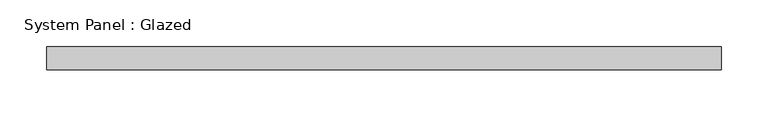
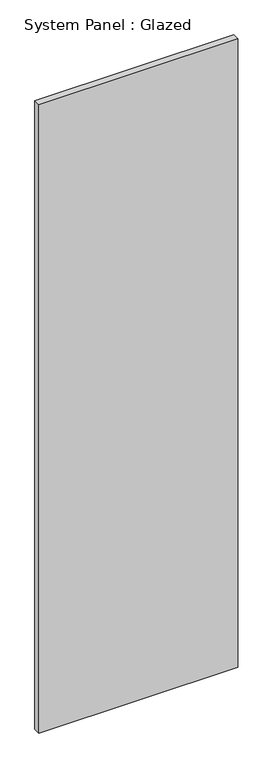
"""IFC4 building model written with IfcOpenShell, lengths in millimetres: plate geometry, System Panel : Glazed."""

from ifc_helpers import new_model, si_unit, origin, origin_with_axes, place, context, project, spatial, polyline, outline, extrude, source, transform, mapped, element, save


def system_panel_glazed_82eb6eb7(model_context):
    return source(origin(), model_context, "Body", "SweptSolid", [
        extrude(outline(polyline([(362.5, 24.5), (-362.5, 24.5), (-362.5, 49.5), (362.5, 49.5), (362.5, 24.5)])), origin_with_axes(), (0.0, 0.0, 1.0), 2422.0),
    ])


if __name__ == "__main__":
    model = new_model("IFC4")
    model_context = context("Model", 3, world=origin())
    ifc_project = project(units=[si_unit("LENGTHUNIT", "METRE", prefix="MILLI")], contexts=[model_context])
    site = spatial("IfcSite", under=ifc_project)
    building = spatial("IfcBuilding", under=site)
    placement = place(None, origin())
    system_panel_glazed_shape = system_panel_glazed_82eb6eb7(model_context)
    element("IfcPlate", 1, ObjectType="System Panel : Glazed", at=placement, inside=building, context=model_context, shape_type="MappedRepresentation", body=[
        mapped(system_panel_glazed_shape, transform((0.0, 0.0, 0.0), x_axis=(1.0, 0.0, 0.0), y_axis=(0.0, 1.0, 0.0), z_axis=(0.0, 0.0, 1.0))),
    ])
    save(model, "model.ifc")

# Revit data of these elements
# Type "System Panel : Glazed"
#   Keynote = "H11"
#   Construction Type Id = "GSP4R"
#   Analytic Construction = "1/8 in Pilkington single glazing"
#   Visual Light Transmittance = 0.9
#   Solar Heat Gain Coefficient = 0.86
#   Heat Transfer Coefficient (U) = 6.7069 W/(m²·K)
#   Define Thermal Properties by = 1
# Element 1 (IfcPlate, "System Panel : Glazed")
#   Materials on its faces: "Glass"
# Materials
#   "Glass": class "Glass", colour RGB 0 128 192, transparency 0.9, Description = "Soda Lime Glass", Cost = 0
